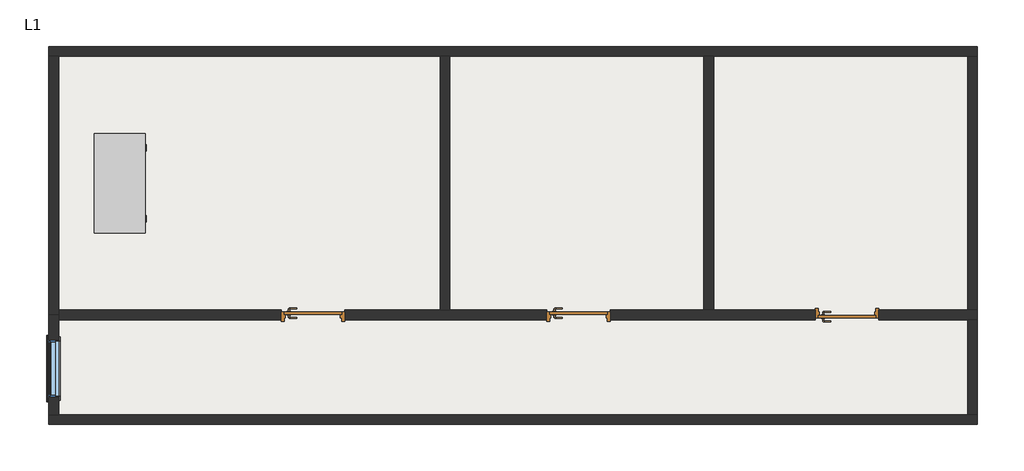
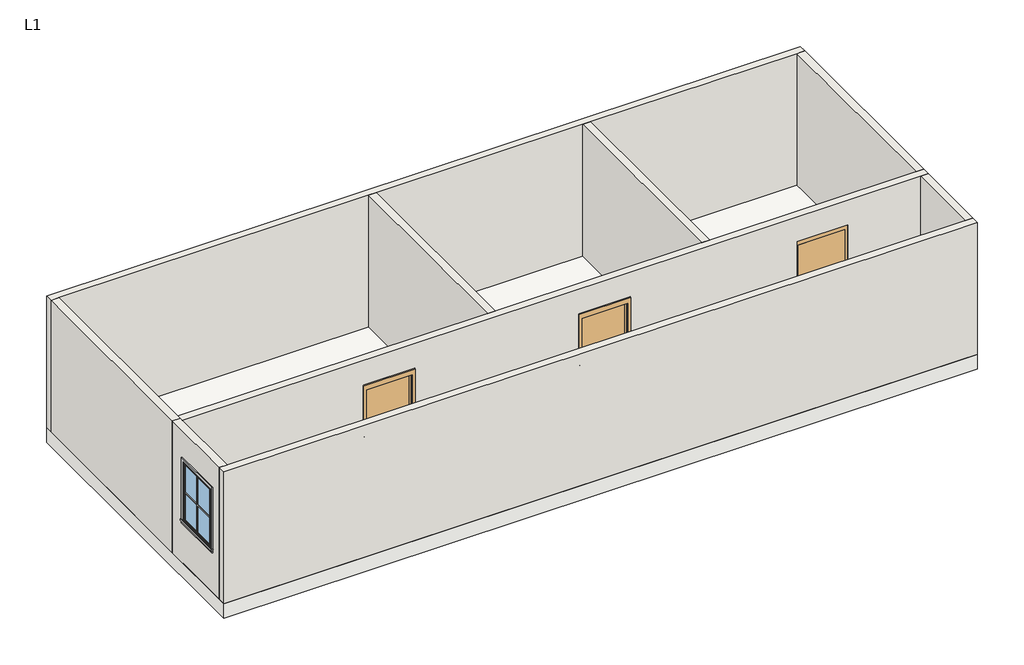
# One storey: 9 walls, 3 doors, 3 proxies, 1 furniture element, 1 slab, 1 window.
# Revit data of these elements (continued)
# Type "M_Trim-Window-Exterior-Flat : with Sill"
#   Trim Width = 60 mm
#   Trim Thickness_Picture Frame = 30 mm
#   Trim Thickness_with Sill = 19.05 mm
#   Sill Thickness = 30 mm
#   Opening Width [instance default] = 600 mm
#   Opening Height [instance default] = 900 mm
#   Default Elevation = 1200 mm
#   Sill = yes
#   Picture Frame = no
#   Trim Material [instance default] = none
# Type "M_Trim-Window-Interior-Flat : Picture Frame"
#   Trim Thickness_Picture Frame = 30 mm
#   Trim Width = 60 mm
#   Trim Thickness_with Sill = 20 mm
#   Sill Thickness = 30 mm
#   Opening Width [instance default] = 600 mm
#   Opening Height [instance default] = 900 mm
#   Default Elevation = 1200 mm
#   Sill = no
#   Picture Frame = yes
#   Trim Material [instance default] = none
# Type "M_Door-Passage-Single-Flush : 900 x 2100mm"
#   Type Mark = "38"
#   Analytic Construction = "Wooden"
#   Thickness = 45 mm
#   Thermal Resistance (R) = 0.455703 (m²·K)/W
#   Swing Angle [instance default] = 90.00°
#   Strike Height = 1000 mm
#   Rough Width [instance default] = 1000 mm
#   Rough Height [instance default] = 2200 mm
#   MF Opening Height [instance default] = 100 mm
#   MF Opening Width [instance default] = 100 mm
#   Inset Calculate [instance default] = 105 mm
#   Masonry Inset [instance default] = 25 mm
#   Height = 2100 mm
#   Width = 900 mm
#   Heat Transfer Coefficient (U) = 2.19465 W/(m²·K)
#   Masonry Frame Depth = 150 mm
#   Masonry Frame [instance default] = yes
#   Function = 1
#   Dry Wall Frame [instance default] = no
#   Panel Material = Wood - Birch
#   Frame Material = Metal - Paint Finish - Grey
#   Door Handle Material = Aluminum
#   Visual Light Transmittance = 0
#   Solar Heat Gain Coefficient = 0
#   Wall Closure = (empty or 0)
# Type "M_Desk : 1525 x 762mm Student"
#   Depth = 762 mm
#   Height = 762 mm
#   Leg Height = 152 mm
#   Width = 1525 mm
#   Body Material = Laminate, Ivory, Matte
#   Handle/Leg Material = Steel, Chrome Plated
#   Top Material = Cherry
#   Default Elevation = 0
# Type "Generic 300mm"
#   Description = "Generic Floor (Material By Category), 300mm thick"
#   Function = 0
#   Layers, outside or top first: 300 mm no material (function 1)
# Type "Generic - 150mm"
#   Description = "Generic Wall (Material By Category), 150mm thick"
#   Type Mark = "G04"
#   Layers, outside or top first: 150 mm no material (function 1)
# Type "M_Window-Fixed : 900 x 1200mm"
#   Type Mark = "36"
#   Fire Rating = "0.5h"
#   Analytic Construction = "Double glazing - domestic"
#   Window Inset [instance default] = 0 mm
#   Wall Thickness [instance default] = 150 mm
#   Visual Light Transmittance = 0.81
#   Thermal Resistance (R) = 0.319569 (m²·K)/W
#   Solar Heat Gain Coefficient = 0.76
#   Rough Width = 915 mm
#   Rough Height = 1215 mm
#   Interior Wall Closure [instance default] = 54.75 mm
#   Height = 1200 mm
#   Heat Transfer Coefficient (U) = 3.12929 W/(m²·K)
#   Frame Extension [instance default] = 6.35 mm
#   Exterior Wall Closure [instance default] = 31.75 mm
#   Extension Jamb [instance default] = 54.75 mm
#   Default Sill Height = 900 mm
#   Width = 900 mm
#   Muntin Visibility = yes
#   Interior Trim Visibility [instance default] = yes
#   Exterior Trim Visibility [instance default] = yes
#   Extension Jamb Visibility [instance default] = yes
#   Muntin Pattern = M_Muntin Pattern_2x2 : M_Muntin Pattern_2x2
#   Interior Trim Material = Wood - Stained
#   Interior Trim = M_Trim-Window-Interior-Flat : Picture Frame
#   Interior Frame Material = Wood - Stained
#   Glass Panel Material = Glass
#   Exterior Trim Material = Clad - White
#   Exterior Trim = M_Trim-Window-Exterior-Flat : with Sill
#   Exterior Frame Material = Clad - White
#   Wall Closure = (empty or 0)
# Element 1 (IfcBuildingElementProxy, "M_Muntin Pattern_2x2 : M_Muntin Pattern_2x2")
#   Width = 823.8 mm
#   Height = 1123.8 mm
#   Interior Material = Wood - Stained
#   Exterior Material = Clad - White
#   Phase Created = New Construction
#   Materials on its faces: "Clad - White", "Wood - Stained"
# Element 2 (IfcBuildingElementProxy, "M_Trim-Window-Exterior-Flat : with Sill")
#   Opening Width = 900 mm
#   Opening Height = 1200 mm
#   Trim Material = Clad - White
#   Phase Created = New Construction
#   Materials on its faces: "Clad - White"
# Element 3 (IfcBuildingElementProxy, "M_Trim-Window-Interior-Flat : Picture Frame")
#   Opening Width = 900 mm
#   Opening Height = 1200 mm
#   Trim Material = Wood - Stained
#   Phase Created = New Construction
#   Materials on its faces: "Wood - Stained"
# Elements 4, 5, 6 (IfcDoor, "M_Door-Passage-Single-Flush : 900 x 2100mm")
#   Swing Angle = 90.00°
#   Rough Width = 1000 mm
#   Rough Height = 2200 mm
#   Masonry Inset = 25 mm
#   MF Opening Width = 100 mm
#   MF Opening Height = 100 mm
#   Inset Calculate = 105 mm
#   Masonry Frame = yes
#   Dry Wall Frame = no
#   Phase Created = New Construction
#   Materials on its faces: "Aluminum", "Metal - Paint Finish - Grey", "Wood - Birch"
# Element 7 (IfcFurniture, "M_Desk : 1525 x 762mm Student")
#   Phase Created = New Construction
#   Materials on its faces: "Steel, Chrome Plated", "Laminate, Ivory, Matte", "Cherry"
# Element 8 (IfcSlab, "Generic 300mm")
#   Height Offset From Level = 0 mm
#   Phase Created = New Construction
#   Materials on its faces: "Default Floor"
# Elements 9, 10, 11, 12, 13, 14, 15 (IfcWall, "Generic - 150mm")
#   Top Offset = 0 mm
#   Base Offset = 0 mm
#   Unconnected Height = 2700 mm
#   wall height = 2700 mm
#   Phase Created = New Construction
#   Base Constraint = L1
#   Materials on its faces: "Default Wall"
# Elements 16, 17 (IfcWall, "Generic - 150mm")
#   Top Offset = 0 mm
#   Base Offset = 0 mm
#   wall height = 2700 mm
#   Phase Created = New Construction
#   Base Constraint = L1
#   Top Constraint = L2
#   Materials on its faces: "Default Wall"
# Element 18 (IfcWindow, "M_Window-Fixed : 900 x 1200mm")
#   Mark = "109"
#   Window Inset = 0 mm
#   Interior Wall Closure = 54.75 mm
#   Frame Extension = 6.35 mm
#   Exterior Wall Closure = 31.75 mm
#   Interior Trim Visibility = yes
#   Exterior Trim Visibility = yes
#   Phase Created = New Construction
#   Materials on its faces: "Wood - Stained", "Glass", "Clad - White"
# Materials
#   "Wood - Birch": class "Wood", colour RGB 173 132 96, transparency 0, Cost = 0
#   "Metal - Paint Finish - Grey": class "Paint", colour RGB 178 178 178, transparency 0, Cost = 0
#   "Aluminum": class "Metal", colour RGB 244 245 246, transparency 0, Description = "Aluminum 6061", Cost = 0
#   "Laminate, Ivory, Matte": class "Plastic", colour RGB 244 244 244, transparency 0, Description = "Plastic Laminate - Ivory, Matte", Cost = 0
#   "Steel, Chrome Plated": class "Metal", colour RGB 17 17 17, transparency 0, Description = "Chromiuim plated steel", Cost = 0
#   "Cherry": class "Wood", colour RGB 158 77 40, transparency 0, Description = "Prunus Serotina", Cost = 0
#   "Wood - Stained": class "Wood", colour RGB 173 132 96, transparency 0, Cost = 0
#   "Glass": class "Glass", colour RGB 245 245 243, transparency 1, Description = "Soda Lime Glass", Cost = 0
#   "Clad - White": class "Wood", colour RGB 245 245 243, transparency 0, Cost = 0
#   "Default Floor": class "Miscellaneous", colour RGB 128 128 128, transparency 0, Cost = 0
#   "Default Wall": class "Miscellaneous", colour RGB 192 192 192, transparency 0, Cost = 0
# Room at (5883.009, 2260.958) mm, phase "New Construction", upper level "L1", upper offset 3048 mm, lower offset 0 mm
#   Number = "100"
#   Name = "Room Name"
# Room at (2241.563, 2260.958) mm, phase "New Construction", upper level "L1", upper offset 3048 mm, lower offset 0 mm
#   Number = "101"
#   Name = "Room Name"
# Room at (-3200.301, 2260.958) mm, phase "New Construction", upper level "L1", upper offset 3048 mm, lower offset 0 mm
#   Number = "102"
#   Name = "Room Name"
# Room at (1659.473, -757.788) mm, phase "New Construction", upper level "L1", upper offset 3048 mm, lower offset 0 mm
#   Number = "103"
#   Name = "Room Name"
